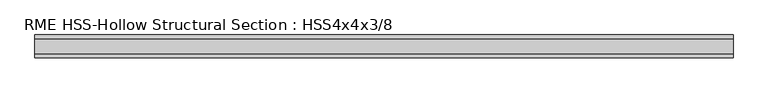
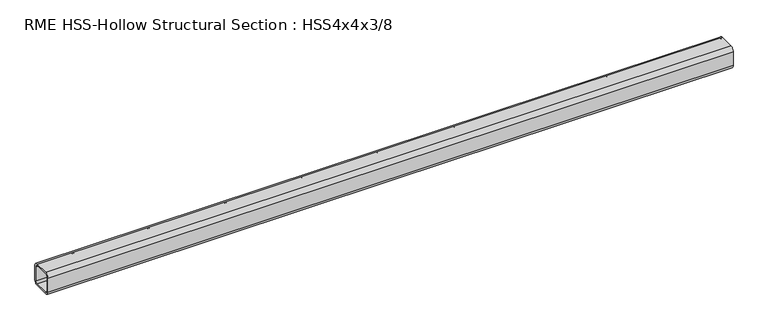
"""IFC4 building model written with IfcOpenShell, lengths in millimetres: member geometry, RME HSS-Hollow Structural Section : HSS4x4x3/8."""

from ifc_helpers import new_model, si_unit, point, frame, frame_2d, origin, place, context, project, spatial, polyline, circle_curve, trimmed, segment, composite_curve, outline, extrude, source, transform, mapped, element, save


def rme_hss_hollow_structural_section_hss4x4x3_8_c9f37aa1(model_context):
    return source(origin(), model_context, "Body", "SweptSolid", [
        extrude(outline(composite_curve([segment(polyline([(50.8, 33.0708), (50.8, -33.0708)]), True, "CONTINUOUS"), segment(trimmed(circle_curve(frame_2d((33.0708, -33.0708)), 17.7292), [point((50.8, -33.0708))], [point((33.0708, -50.8))], False, "CARTESIAN"), True, "CONTINUOUS"), segment(polyline([(33.0708, -50.8), (-33.0708, -50.8)]), True, "CONTINUOUS"), segment(trimmed(circle_curve(frame_2d((-33.0708, -33.0708)), 17.7292), [point((-33.0708, -50.8))], [point((-50.8, -33.0708))], False, "CARTESIAN"), True, "CONTINUOUS"), segment(polyline([(-50.8, -33.0708), (-50.8, 33.0708)]), True, "CONTINUOUS"), segment(trimmed(circle_curve(frame_2d((-33.0708, 33.0708)), 17.7292), [point((-50.8, 33.0708))], [point((-33.0708, 50.8))], False, "CARTESIAN"), True, "CONTINUOUS"), segment(polyline([(-33.0708, 50.8), (33.0708, 50.8)]), True, "CONTINUOUS"), segment(trimmed(circle_curve(frame_2d((33.0708, 33.0708)), 17.7292), [point((33.0708, 50.8))], [point((50.8, 33.0708))], False, "CARTESIAN"), True, "CONTINUOUS")], self_intersect=False), holes=[composite_curve([segment(trimmed(circle_curve(frame_2d((-33.0708, 33.0708)), 8.8646), [point((-33.0708, 41.9354))], [point((-41.9354, 33.0708))], True, "CARTESIAN"), True, "CONTINUOUS"), segment(polyline([(-41.9354, 33.0708), (-41.9354, -33.0708)]), True, "CONTINUOUS"), segment(trimmed(circle_curve(frame_2d((-33.0708, -33.0708)), 8.8646), [point((-41.9354, -33.0708))], [point((-33.0708, -41.9354))], True, "CARTESIAN"), True, "CONTINUOUS"), segment(polyline([(-33.0708, -41.9354), (33.0708, -41.9354)]), True, "CONTINUOUS"), segment(trimmed(circle_curve(frame_2d((33.0708, -33.0708)), 8.8646), [point((33.0708, -41.9354))], [point((41.9354, -33.0708))], True, "CARTESIAN"), True, "CONTINUOUS"), segment(polyline([(41.9354, -33.0708), (41.9354, 33.0708)]), True, "CONTINUOUS"), segment(trimmed(circle_curve(frame_2d((33.0708, 33.0708)), 8.8646), [point((41.9354, 33.0708))], [point((33.0708, 41.9354))], True, "CARTESIAN"), True, "CONTINUOUS"), segment(polyline([(33.0708, 41.9354), (-33.0708, 41.9354)]), True, "CONTINUOUS")], self_intersect=False)]), frame((-1688.8681109, 0.0, 0.0), z_axis=(1.0, 0.0, 0.0), x_axis=(0.0, 1.0, 0.0)), (0.0, 0.0, 1.0), 3086.0159856),
    ])


if __name__ == "__main__":
    model = new_model("IFC4")
    model_context = context("Model", 3, world=origin())
    ifc_project = project(units=[si_unit("LENGTHUNIT", "METRE", prefix="MILLI")], contexts=[model_context])
    site = spatial("IfcSite", under=ifc_project)
    building = spatial("IfcBuilding", under=site)
    placement = place(None, origin())
    rme_hss_hollow_structural_section_hss4x4x3_8_shape = rme_hss_hollow_structural_section_hss4x4x3_8_c9f37aa1(model_context)
    element("IfcMember", 1, ObjectType="RME HSS-Hollow Structural Section : HSS4x4x3/8", at=placement, inside=building, context=model_context, shape_type="MappedRepresentation", body=[
        mapped(rme_hss_hollow_structural_section_hss4x4x3_8_shape, transform((0.0, 0.0, 0.0), x_axis=(1.0, 0.0, 0.0), y_axis=(0.0, 1.0, 0.0), z_axis=(0.0, 0.0, 1.0))),
    ])
    save(model, "model.ifc")

# Revit data of these elements
# Type "RME HSS-Hollow Structural Section : HSS4x4x3/8"
#   Nominal Size = "HSS6x4"
#   Assembly Code = "B10"
#   Shape = "Square"
#   W = 17.2
#   Start Extension Calculation [instance default] = 10' - 0"
#   Start Extension [instance default] = -0' - 0 1/2"
#   End Extension Calculation [instance default] = 10' - 0"
#   End Extension [instance default] = -0' - 0 1/2"
#   Ht = 0' - 4"
#   Length [instance default] = 5' - 0"
#   b = 0' - 4"
#   kr = 0' - 0.698"
#   t = 0' - 0.349"
#   A = 0.0331944 SF
#   Structural Material [instance default] = Metal - Steel - ASTM A500 - Grade B - Rectangular and Square
# Element 1 (IfcMember, "RME HSS-Hollow Structural Section : HSS4x4x3/8")
#   End Extension Calculation = 9' - 8.41105"
#   End Extension = -0' - 4.08895"
#   Structural Material = Metal - Steel - ASTM A992
#   Materials on its faces: "Metal - Steel - ASTM A992"
# Materials
#   "Metal - Steel - ASTM A500 - Grade B - Rectangular and Square": class "Metal", colour RGB 255 128 0, transparency 0
#   "Metal - Steel - ASTM A992": class "Metal", colour RGB 255 128 0, transparency 0
